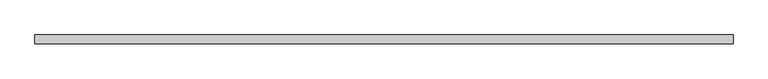
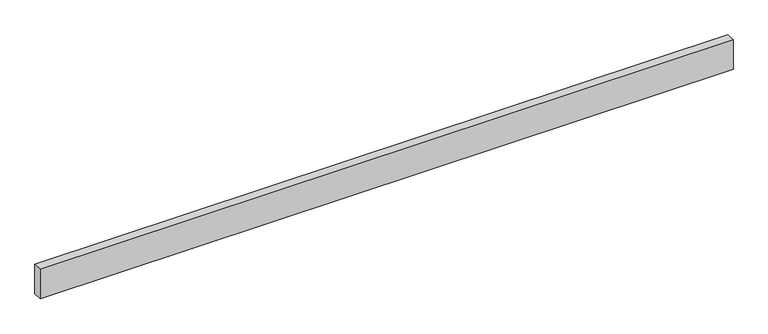
"""IFC4 building model written with IfcOpenShell, lengths in millimetres: beam geometry, NLRS_28_SF_LIB_houten balk-MMBW-SRP_gen_rsf : houten balk_gen__bxh 70x195."""

import ifcopenshell
import ifcopenshell.guid

model = None  # the IFC model being written
_history = None  # IfcOwnerHistory: only IFC2X3 demands one
_inside = {}  # id of a spatial element -> (the spatial element, [elements in it])
_under = {}  # id of a project, library or spatial element -> (it, [spatial elements below it])
_declared = {}  # id of a project -> (the project, [libraries it declares])
_typed = {}  # id of a type object -> (the type object, [elements of that type])
_made_of = {}  # id of a material, layer set ... -> (it, [elements and type objects made of it])


def new_model(schema):
    """Start an empty IFC model of exactly this schema.

    Asked for "IFC4X3", IfcOpenShell would pick the latest addendum, in which some entities
    have other attributes; the version numbers below select the first issue.
    IFC2X3 requires an IfcOwnerHistory on every rooted entity: one is made here for all.
    """
    global model, _history
    if schema == "IFC4X3":
        model = ifcopenshell.file(schema_version=(4, 3, 0, 0))
    else:
        model = ifcopenshell.file(schema=schema)
    _inside.clear()
    _under.clear()
    _declared.clear()
    _typed.clear()
    _made_of.clear()
    _history = None
    if model.schema == "IFC2X3":
        org = make("IfcOrganization", Name="unknown")
        user = make(
            "IfcPersonAndOrganization",
            ThePerson=make("IfcPerson", FamilyName="unknown"),
            TheOrganization=org,
        )
        app = make(
            "IfcApplication",
            ApplicationDeveloper=org,
            Version="unknown",
            ApplicationFullName="unknown",
            ApplicationIdentifier="unknown",
        )
        _history = make(
            "IfcOwnerHistory",
            OwningUser=user,
            OwningApplication=app,
            ChangeAction="ADDED",
            CreationDate=0,
        )
    return model


def make(cls, **values):
    """One entity of the class cls with the attributes given. An attribute that is None is left unset."""
    return model.create_entity(
        cls, **{name: value for name, value in values.items() if value is not None}
    )


def rooted(cls, **values):
    """An entity with a GlobalId (a new one), such as an element, a storey or a relation."""
    return make(cls, GlobalId=ifcopenshell.guid.new(), OwnerHistory=_history, **values)


def si_unit(unit_type, name, prefix=None):
    """IfcSIUnit, for example si_unit("LENGTHUNIT", "METRE", prefix="MILLI")."""
    return make("IfcSIUnit", UnitType=unit_type, Prefix=prefix, Name=name)


def assignment(units):
    """IfcUnitAssignment: the units of a project."""
    return None if units is None else make("IfcUnitAssignment", Units=units)


def point(xyz):
    """IfcCartesianPoint."""
    return None if xyz is None else make("IfcCartesianPoint", Coordinates=xyz)


def direction(xyz):
    """IfcDirection."""
    return None if xyz is None else make("IfcDirection", DirectionRatios=xyz)


def frame(location, z_axis=None, x_axis=None):
    """IfcAxis2Placement3D, a coordinate frame: its origin and axes. An axis left out is left unset."""
    return make(
        "IfcAxis2Placement3D",
        Location=point(location),
        Axis=direction(z_axis),
        RefDirection=direction(x_axis),
    )


def origin():
    """The frame at (0, 0, 0) with its axes left unset."""
    return frame((0.0, 0.0, 0.0))


def place(relative_to, where):
    """IfcLocalPlacement: puts the frame where relative to a parent placement (None: the world)."""
    return make(
        "IfcLocalPlacement", PlacementRelTo=relative_to, RelativePlacement=where
    )


def context(
    kind, dimensions, precision=None, world=None, true_north=None, identifier=None
):
    """IfcGeometricRepresentationContext, for example the 3D "Model" context."""
    return make(
        "IfcGeometricRepresentationContext",
        ContextIdentifier=identifier,
        ContextType=kind,
        CoordinateSpaceDimension=dimensions,
        Precision=precision,
        WorldCoordinateSystem=world,
        TrueNorth=true_north,
    )


def project(units=None, contexts=None):
    """IfcProject with its units and contexts."""
    return rooted(
        "IfcProject",
        Name="project",
        RepresentationContexts=contexts,
        UnitsInContext=assignment(units),
    )


def spatial(cls, under=None, at=None, **own):
    """A site, building, storey or space (cls), placed at a placement, below another one or the project."""
    s = rooted(cls, ObjectPlacement=at, **own)
    if under is not None:
        _under.setdefault(under.id(), (under, []))[1].append(s)
    return s


def polyline(points):
    """IfcPolyline through the points."""
    return make("IfcPolyline", Points=[point(p) for p in points])


def outline(outer, holes=None, kind="AREA"):
    """IfcArbitraryClosedProfileDef: a profile drawn as a closed curve; with holes, ...WithVoids."""
    if holes is None:
        return make("IfcArbitraryClosedProfileDef", ProfileType=kind, OuterCurve=outer)
    return make(
        "IfcArbitraryProfileDefWithVoids",
        ProfileType=kind,
        OuterCurve=outer,
        InnerCurves=holes,
    )


def extrude(swept, where, along, depth):
    """IfcExtrudedAreaSolid: the profile swept, set in the frame where, extruded along a direction by depth."""
    return make(
        "IfcExtrudedAreaSolid",
        SweptArea=swept,
        Position=where,
        ExtrudedDirection=direction(along),
        Depth=depth,
    )


def shape(context_of_items, identifier, shape_type, items):
    """IfcShapeRepresentation: the items that make up one representation, for example the "Body"."""
    return make(
        "IfcShapeRepresentation",
        ContextOfItems=context_of_items,
        RepresentationIdentifier=identifier,
        RepresentationType=shape_type,
        Items=items,
    )


def source(mapping_origin, context_of_items, identifier, shape_type, items):
    """IfcRepresentationMap: a shape defined once, which mapped items show again and again."""
    return make(
        "IfcRepresentationMap",
        MappingOrigin=mapping_origin,
        MappedRepresentation=shape(context_of_items, identifier, shape_type, items),
    )


def transform(
    local_origin,
    x_axis=None,
    y_axis=None,
    z_axis=None,
    scale=None,
    scale2=None,
    scale3=None,
    uniform=True,
):
    """IfcCartesianTransformationOperator3D, or its non-uniform kind. x_axis, y_axis, z_axis: its Axis1, 2, 3."""
    if uniform:
        return make(
            "IfcCartesianTransformationOperator3D",
            Axis1=direction(x_axis),
            Axis2=direction(y_axis),
            LocalOrigin=point(local_origin),
            Scale=scale,
            Axis3=direction(z_axis),
        )
    return make(
        "IfcCartesianTransformationOperator3DnonUniform",
        Axis1=direction(x_axis),
        Axis2=direction(y_axis),
        LocalOrigin=point(local_origin),
        Scale=scale,
        Axis3=direction(z_axis),
        Scale2=scale2,
        Scale3=scale3,
    )


def mapped(mapping_source, mapping_target):
    """IfcMappedItem: shows the shape of a source again, moved by a transform."""
    return make(
        "IfcMappedItem", MappingSource=mapping_source, MappingTarget=mapping_target
    )


def made_of(thing, what):
    """Note that an element or type object is made of a material, layer set ...; save() writes the relation."""
    if what is not None:
        _made_of.setdefault(what.id(), (what, []))[1].append(thing)
    return thing


def element(
    cls,
    number,
    at=None,
    inside=None,
    cuts=None,
    type_object=None,
    material=None,
    context=None,
    identifier="Body",
    shape_type=None,
    held_by="IfcProductDefinitionShape",
    body=None,
    shapes=None,
    **own,
):
    """One element of the class cls, such as IfcWall. Its Tag is "e" and its number.

    at: its placement. inside: the storey or other place that contains it. cuts: it is an
    opening in that element (IfcRelVoidsElement). A single representation is given by context,
    identifier, shape_type and body (its items); several are given by shapes. held_by: the class
    of the entity that holds the representations. save() writes the other relations.
    """
    e = rooted(cls, Tag="e%d" % number, ObjectPlacement=at, **own)
    if body is not None:
        shapes = [shape(context, identifier, shape_type, body)]
    if shapes is not None:
        e.Representation = make(held_by, Representations=shapes)
    if inside is not None:
        _inside.setdefault(inside.id(), (inside, []))[1].append(e)
    if cuts is not None:
        rooted(
            "IfcRelVoidsElement", RelatingBuildingElement=cuts, RelatedOpeningElement=e
        )
    if type_object is not None:
        _typed.setdefault(type_object.id(), (type_object, []))[1].append(e)
    return made_of(e, material)


def aggregate(whole, parts):
    """IfcRelAggregates: a whole, such as a stair, and the parts it consists of."""
    return rooted("IfcRelAggregates", RelatingObject=whole, RelatedObjects=parts)


def save(model, path):
    """Write the relations noted so far, then the file.

    IfcRelAggregates (storeys below a building ...), IfcRelContainedInSpatialStructure (elements
    in a storey), IfcRelDefinesByType, IfcRelAssociatesMaterial and IfcRelDeclares: one each for
    every whole, place, type object, material and project.
    """
    for whole, parts in _under.values():
        aggregate(whole, parts)
    for where, things in _inside.values():
        rooted(
            "IfcRelContainedInSpatialStructure",
            RelatedElements=things,
            RelatingStructure=where,
        )
    for kind, things in _typed.values():
        rooted("IfcRelDefinesByType", RelatedObjects=things, RelatingType=kind)
    for what, things in _made_of.values():
        rooted("IfcRelAssociatesMaterial", RelatedObjects=things, RelatingMaterial=what)
    for by, libraries in _declared.values():
        rooted("IfcRelDeclares", RelatingContext=by, RelatedDefinitions=libraries)
    model.write(path)


def beam_9365c9be(model_context):
    return source(origin(), model_context, "Body", "SweptSolid", [
        extrude(outline(polyline([(-2751.0, -35.0), (-2751.0, 35.0), (2751.0, 35.0), (2751.0, -35.0), (-2751.0, -35.0)])), frame((0.0, 0.0, -122.5), z_axis=(0.0, 0.0, 1.0), x_axis=(1.0, 0.0, 0.0)), (0.0, 0.0, 1.0), 245.0),
    ])


if __name__ == "__main__":
    model = new_model("IFC4")
    model_context = context("Model", 3, world=origin())
    ifc_project = project(units=[si_unit("LENGTHUNIT", "METRE", prefix="MILLI")], contexts=[model_context])
    site = spatial("IfcSite", under=ifc_project)
    building = spatial("IfcBuilding", under=site)
    placement = place(None, origin())
    beam_shape = beam_9365c9be(model_context)
    element("IfcBeam", 1, ObjectType="NLRS_28_SF_LIB_houten balk-MMBW-SRP_gen_rsf : houten balk_gen__bxh 70x195", at=placement, inside=building, context=model_context, shape_type="MappedRepresentation", body=[
        mapped(beam_shape, transform((0.0, 0.0, 0.0), x_axis=(1.0, 0.0, 0.0), y_axis=(0.0, 1.0, 0.0), z_axis=(0.0, 0.0, 1.0))),
    ])
    save(model, "model.ifc")

# Revit data of these elements
# Type "NLRS_28_SF_LIB_houten balk-MMBW-SRP_gen_rsf : houten balk_gen__bxh 70x195"
#   Type IfcGUID = "07M7mRoiH1CR8m_RSKIvYS"
#   IfcExportAs = "IfcBeamType"
#   Type Comments = "70x195"
#   Model = " "
#   Manufacturer = " "
#   Fire Rating = " "
#   Description = "houten balk 70x195"
#   Assembly Code = "28.11"
#   NLRS_C_lengte [instance default] = 3000 mm
#   NLRS_C_hoogte = 245 mm
#   NLRS_C_breedte = 70 mm
#   Length [instance default] = 3000 mm
#   Structural Material = NLRS_i2_hout naaldhout vuren_gen_rsf
#   Keynote = ""
# Element 1 (IfcBeam, "NLRS_28_SF_LIB_houten balk-MMBW-SRP_gen_rsf : houten balk_gen__bxh 70x195")
#   NLRS_C_lengte = 5572 mm
#   Materials on its faces: "NLRS_i2_hout naaldhout vuren_gen_rsf"
# Materials
#   "NLRS_i2_hout naaldhout vuren_gen_rsf": class "I - Hout", colour RGB 234 199 147, transparency 0, Keynote = "i2", Manufacturer = "Revit Standards Foundation", URL = "www.revitstandards.org", Description = "hout vuren", Cost = 0
